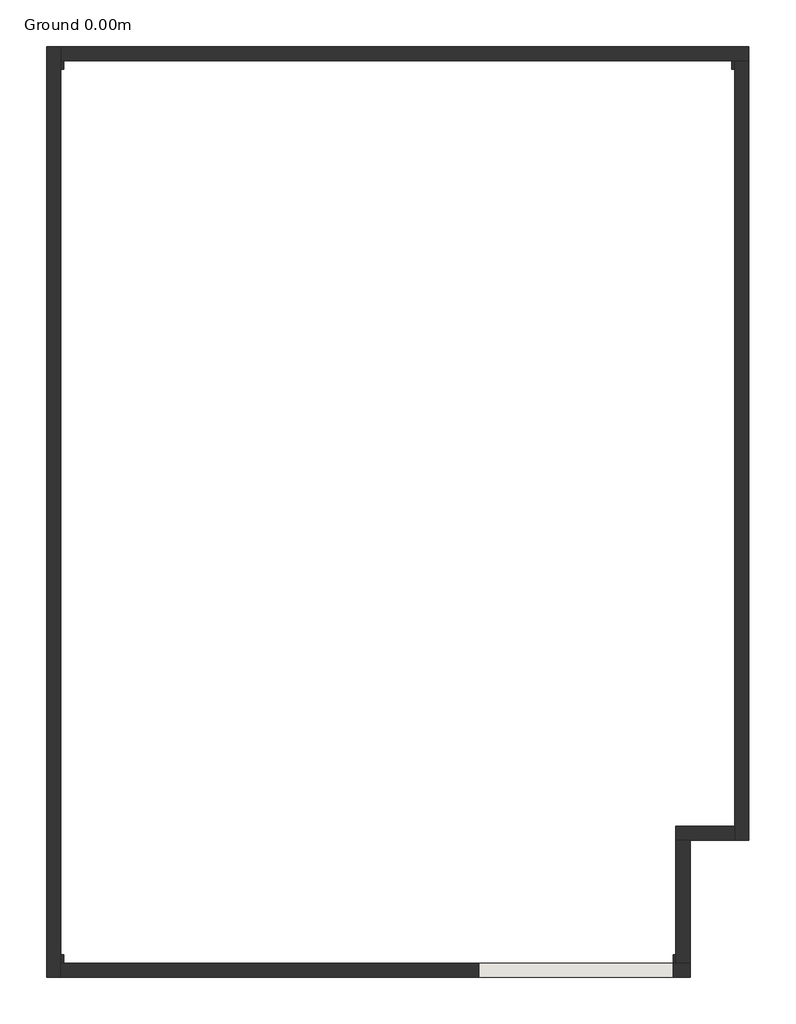
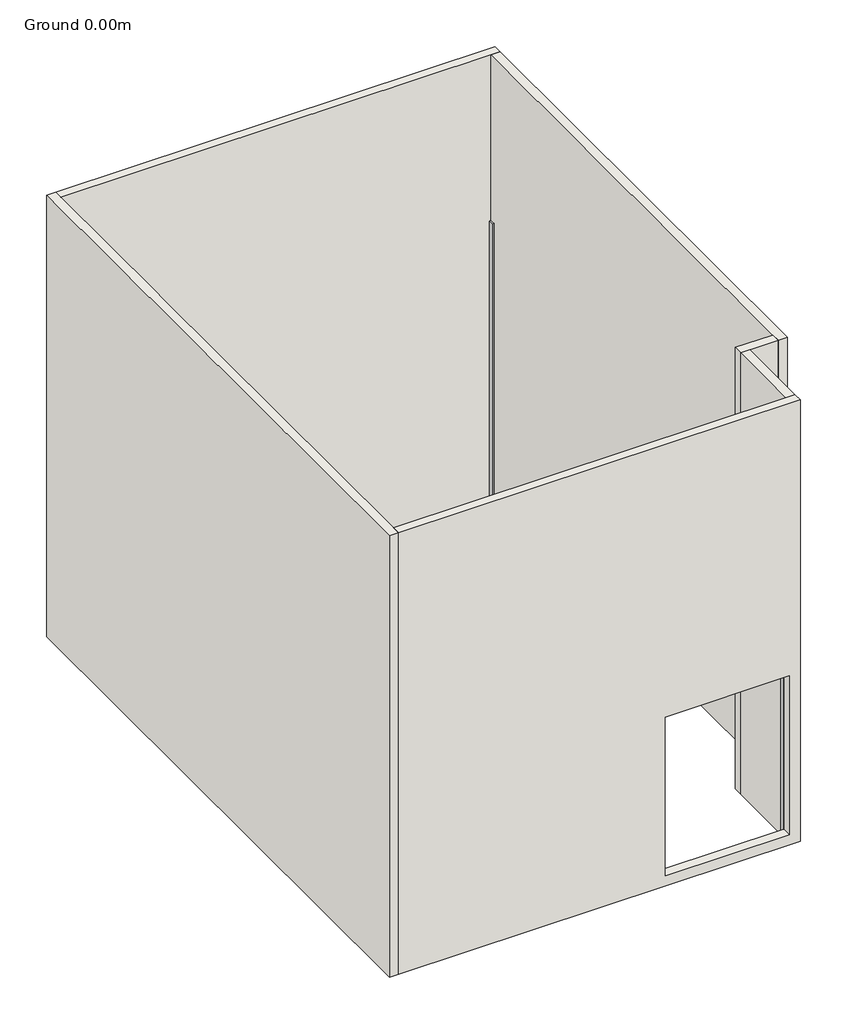
# One storey: 6 walls, 4 columns.
"""IFC4 building model written with IfcOpenShell, lengths in millimetres."""

from ifc_helpers import new_model, si_unit, origin, origin_with_axes, place, context, project, spatial, polyline, outline, extrude, faceted_brep, element, save

model = new_model("IFC4")

# Units and contexts
model_context = context("Model", 3, world=origin())
ifc_project = project(units=[si_unit("LENGTHUNIT", "METRE", prefix="MILLI")], contexts=[model_context])

# Site, building, storey
site = spatial("IfcSite", under=ifc_project)
building = spatial("IfcBuilding", under=site)
storey = spatial("IfcBuildingStorey", under=building, Name="Ground 0.00m", Elevation=0.0)

# Columns
placement = place(None, origin())
element("IfcColumn", 1, ObjectType="Columns_Rectangular : 150 X 200", at=placement, inside=storey, context=model_context, shape_type="SweptSolid", body=[
    extrude(outline(polyline([(-3078.7164348, 3857.7470308), (-3103.7164348, 3857.7470308), (-3103.7164348, 3932.7470308), (-3078.7164348, 3932.7470308), (-3078.7164348, 3857.7470308)])), origin_with_axes(), (0.0, 0.0, 1.0), 4000.0),
])
element("IfcColumn", 2, ObjectType="Columns_Rectangular : 150 X 200", at=placement, inside=storey, context=model_context, shape_type="SweptSolid", body=[
    extrude(outline(polyline([(-3103.7164348, -3892.2529692), (-3078.7164348, -3892.2529692), (-3078.7164348, -3967.2529692), (-3103.7164348, -3967.2529692), (-3103.7164348, -3892.2529692)])), origin_with_axes(), (0.0, 0.0, 1.0), 4000.0),
])
element("IfcColumn", 3, ObjectType="Columns_Rectangular : 150 X 200", at=placement, inside=storey, context=model_context, shape_type="Brep", body=[
    faceted_brep([(2256.2835652, -3892.2529692, 4000.0), (2256.2835652, -3967.2529692, 4000.0), (2281.2835652, -3967.2529692, 4000.0), (2281.2835652, -3892.2529692, 4000.0), (2256.2835652, -3967.2529692, 0.0), (2256.2835652, -3892.2529692, 0.0), (2281.2835652, -3892.2529692, 0.0), (2281.2835652, -3967.2529692, 0.0), (2256.2835652, -3967.2529692, 150.0), (2256.2835652, -3967.2529692, 2450.0)], [[[0, 1, 2, 3]], [[4, 5, 6, 7]], [[0, 5, 4, 8, 9, 1]], [[5, 0, 3, 6]], [[1, 9, 8, 4, 7, 2]], [[3, 2, 7, 6]]]),
])
element("IfcColumn", 4, ObjectType="Columns_Rectangular : 150 X 200", at=placement, inside=storey, context=model_context, shape_type="SweptSolid", body=[
    extrude(outline(polyline([(2771.2835652, 3857.7470308), (2771.2835652, 3932.7470308), (2796.2835652, 3932.7470308), (2796.2835652, 3857.7470308), (2771.2835652, 3857.7470308)])), origin_with_axes(), (0.0, 0.0, 1.0), 4000.0),
])

# Walls
element("IfcWall", 5, ObjectType="Wall-Int_12P-100Blk-12P", at=placement, inside=storey, context=model_context, shape_type="Brep", body=[
    faceted_brep([(-3103.7164348, -4092.2529692, 0.0), (-3103.7164348, -3967.2529692, 0.0), (-3103.7164348, -3892.2529692, 0.0), (-3103.7164348, 3857.7470308, 0.0), (-3103.7164348, 3932.7470308, 0.0), (-3103.7164348, 4057.7470308, 0.0), (-3103.7164348, 4057.7470308, 6400.0), (-3103.7164348, 3932.7470308, 6400.0), (-3103.7164348, 1657.7470308, 6400.0), (-3103.7164348, 1532.7470308, 6400.0), (-3103.7164348, -3967.2529692, 6400.0), (-3103.7164348, -4092.2529692, 6400.0), (-3228.7164348, -4092.2529692, 0.0), (-3228.7164348, -4092.2529692, 6400.0), (-3228.7164348, 4057.7470308, 6400.0), (-3228.7164348, 4057.7470308, 0.0)], [[[0, 1, 2, 3, 4, 5, 6, 7, 8, 9, 10, 11]], [[12, 13, 14, 15]], [[5, 4, 3, 2, 1, 0, 12, 15]], [[11, 10, 9, 8, 7, 6, 14, 13]], [[6, 5, 15, 14]], [[0, 11, 13, 12]]]),
])
element("IfcWall", 6, ObjectType="Wall-Int_12P-100Blk-12P", at=placement, inside=storey, context=model_context, shape_type="Brep", body=[
    faceted_brep([(-3103.7164348, 3932.7470308, 0.0), (-3078.7164348, 3932.7470308, 0.0), (2771.2835652, 3932.7470308, 0.0), (2796.2835652, 3932.7470308, 0.0), (2921.2835652, 3932.7470308, 0.0), (2921.2835652, 3932.7470308, 6400.0), (2796.2835652, 3932.7470308, 6400.0), (-3103.7164348, 3932.7470308, 6400.0), (-3103.7164348, 3932.7470308, 4000.0), (-3103.7164348, 4057.7470308, 0.0), (-3103.7164348, 4057.7470308, 6400.0), (2921.2835652, 4057.7470308, 6400.0), (2921.2835652, 4057.7470308, 0.0)], [[[0, 1, 2, 3, 4, 5, 6, 7, 8]], [[9, 10, 11, 12]], [[4, 3, 2, 1, 0, 9, 12]], [[7, 6, 5, 11, 10]], [[0, 8, 7, 10, 9]], [[5, 4, 12, 11]]]),
])
element("IfcWall", 7, ObjectType="Wall-Int_12P-100Blk-12P", at=placement, inside=storey, context=model_context, shape_type="Brep", body=[
    faceted_brep([(2796.2835652, 3932.7470308, 0.0), (2796.2835652, 3857.7470308, 0.0), (2796.2835652, -2767.2529692, 0.0), (2796.2835652, -2892.2529692, 0.0), (2796.2835652, -2892.2529692, 6400.0), (2796.2835652, -2767.2529692, 6400.0), (2796.2835652, 3932.7470308, 6400.0), (2796.2835652, 3932.7470308, 4000.0), (2921.2835652, 3932.7470308, 0.0), (2921.2835652, 3932.7470308, 6400.0), (2921.2835652, -2892.2529692, 6400.0), (2921.2835652, -2892.2529692, 0.0)], [[[0, 1, 2, 3, 4, 5, 6, 7]], [[8, 9, 10, 11]], [[3, 2, 1, 0, 8, 11]], [[6, 5, 4, 10, 9]], [[0, 7, 6, 9, 8]], [[4, 3, 11, 10]]]),
])
element("IfcWall", 8, ObjectType="Wall-Int_12P-100Blk-12P", at=placement, inside=storey, context=model_context, shape_type="Brep", body=[
    faceted_brep([(2406.2835652, -3967.2529692, 0.0), (2281.2835652, -3967.2529692, 0.0), (2256.2835652, -3967.2529692, 0.0), (-3078.7164348, -3967.2529692, 0.0), (-3103.7164348, -3967.2529692, 0.0), (-3103.7164348, -3967.2529692, 4000.0), (-3103.7164348, -3967.2529692, 6400.0), (2281.2835652, -3967.2529692, 6400.0), (2406.2835652, -3967.2529692, 6400.0), (556.2835652, -3967.2529692, 150.0), (2256.2835652, -3967.2529692, 150.0), (2256.2835652, -3967.2529692, 2450.0), (556.2835652, -3967.2529692, 2450.0), (2406.2835652, -4092.2529692, 0.0), (2406.2835652, -4092.2529692, 6400.0), (-3103.7164348, -4092.2529692, 6400.0), (-3103.7164348, -4092.2529692, 0.0), (556.2835652, -4092.2529692, 150.0), (556.2835652, -4092.2529692, 2450.0), (2256.2835652, -4092.2529692, 2450.0), (2256.2835652, -4092.2529692, 150.0)], [[[0, 1, 2, 3, 4, 5, 6, 7, 8], [9, 10, 11, 12]], [[13, 14, 15, 16], [17, 18, 19, 20]], [[4, 3, 2, 1, 0, 13, 16]], [[8, 7, 6, 15, 14]], [[6, 5, 4, 16, 15]], [[18, 17, 9, 12]], [[19, 18, 12, 11]], [[20, 19, 11, 10]], [[17, 20, 10, 9]], [[0, 8, 14, 13]]]),
])
element("IfcWall", 9, ObjectType="Wall-Int_12P-100Blk-12P", at=placement, inside=storey, context=model_context, shape_type="Brep", body=[
    faceted_brep([(2796.2835652, -2767.2529692, 0.0), (2281.2835652, -2767.2529692, 0.0), (2281.2835652, -2767.2529692, 6400.0), (2796.2835652, -2767.2529692, 6400.0), (2796.2835652, -2892.2529692, 0.0), (2796.2835652, -2892.2529692, 6400.0), (2406.2835652, -2892.2529692, 6400.0), (2281.2835652, -2892.2529692, 6400.0), (2281.2835652, -2892.2529692, 0.0), (2406.2835652, -2892.2529692, 0.0)], [[[0, 1, 2, 3]], [[4, 5, 6, 7, 8, 9]], [[1, 0, 4, 9, 8]], [[3, 2, 7, 6, 5]], [[0, 3, 5, 4]], [[2, 1, 8, 7]]]),
])
element("IfcWall", 10, ObjectType="Wall-Int_12P-100Blk-12P", at=placement, inside=storey, context=model_context, shape_type="Brep", body=[
    faceted_brep([(2281.2835652, -2892.2529692, 0.0), (2281.2835652, -3892.2529692, 0.0), (2281.2835652, -3967.2529692, 0.0), (2281.2835652, -3967.2529692, 4000.0), (2281.2835652, -3967.2529692, 6400.0), (2281.2835652, -2892.2529692, 6400.0), (2406.2835652, -2892.2529692, 0.0), (2406.2835652, -2892.2529692, 6400.0), (2406.2835652, -3967.2529692, 6400.0), (2406.2835652, -3967.2529692, 0.0)], [[[0, 1, 2, 3, 4, 5]], [[6, 7, 8, 9]], [[2, 1, 0, 6, 9]], [[5, 4, 8, 7]], [[0, 5, 7, 6]], [[4, 3, 2, 9, 8]]]),
])

save(model, "model.ifc")

# Revit data of these elements
# Project information
#   Project Issue Date = "Issue Date"
#   Project Status = "Project Status"
#   Client Name = "Owner"
#   Project Address = "Enter address here"
#   Project Name = "Project Name"
#   Project Number = "Project Number"
# Grids (mm)
#   "1": line (4318.976, 3932.747) -> (-4543.204, 3932.747)
#   "A": line (-3103.716, -5877.781) -> (-3103.716, 5672.327)
#   "B": line (2796.284, -5877.781) -> (2796.284, 5672.327)
#   "2": line (4318.976, -3967.253) -> (-4543.204, -3967.253)
# Type "Columns_Rectangular : 150 X 200"
#   Depth = 150 mm
#   Offset Base = 0 mm
#   Offset Top = 0 mm
#   Width = 200 mm
#   Material = none
# Type "Wall-Int_12P-100Blk-12P"
#   Layers, outside or top first: 12.5 mm "Plaster" (function 5); 100 mm "Concrete Masonry Units" (function 1); 12.5 mm "Plaster" (function 5)
# Elements 1, 2, 3, 4 (IfcColumn, "Columns_Rectangular : 150 X 200")
#   Phase Created = New Construction
#   Materials on its faces: "Plaster"
# Elements 5, 6, 7, 9 (IfcWall, "Wall-Int_12P-100Blk-12P")
#   Top Offset = 0 mm
#   Base Offset = 0 mm
#   Unconnected Height = 6400 mm
#   wall height = 6400 mm
#   Phase Created = New Construction
#   Base Constraint = Ground 0.00m
#   Materials on its faces: "Plaster", "Default Wall"
# Elements 8, 10 (IfcWall, "Wall-Int_12P-100Blk-12P")
#   Top Offset = 0 mm
#   Base Offset = 0 mm
#   Unconnected Height = 6400 mm
#   wall height = 6400 mm
#   Phase Created = New Construction
#   Base Constraint = Ground 0.00m
#   Materials on its faces: "Default Wall", "Plaster"
# Materials
#   "Plaster": class "Generic", colour RGB 249 249 249, transparency 0, Description = "Plaster", Cost = 0
#   "Concrete Masonry Units": class "Masonry", colour RGB 181 181 181, transparency 0, Description = "Concrete masonry units", Cost = 0
#   "Default Wall": class "Miscellaneous", colour RGB 128 128 128, transparency 0, Comments = "Rendering appearance not upgraded ", Cost = 0
